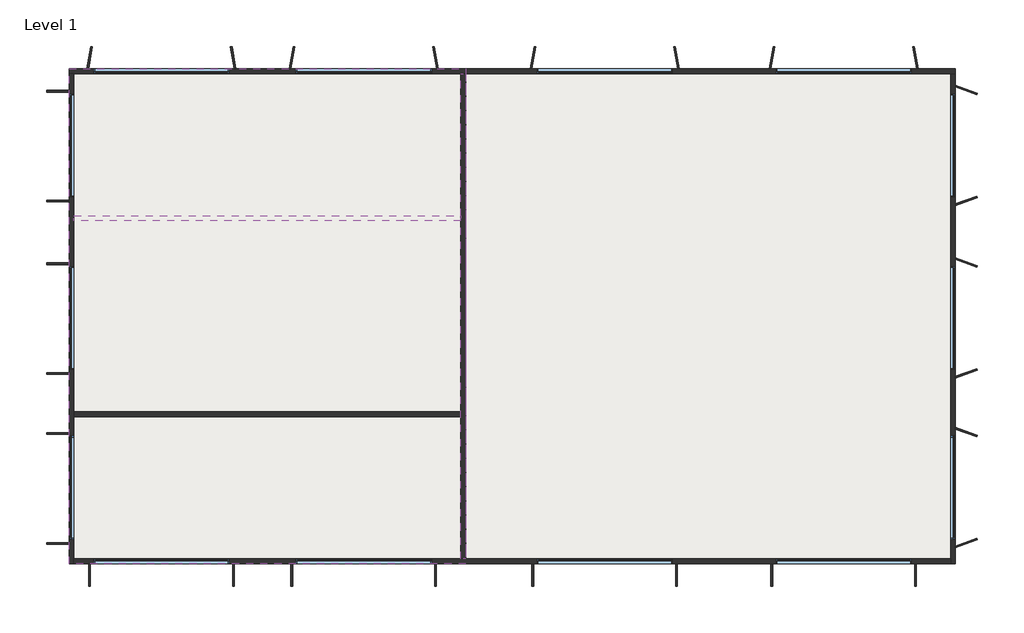
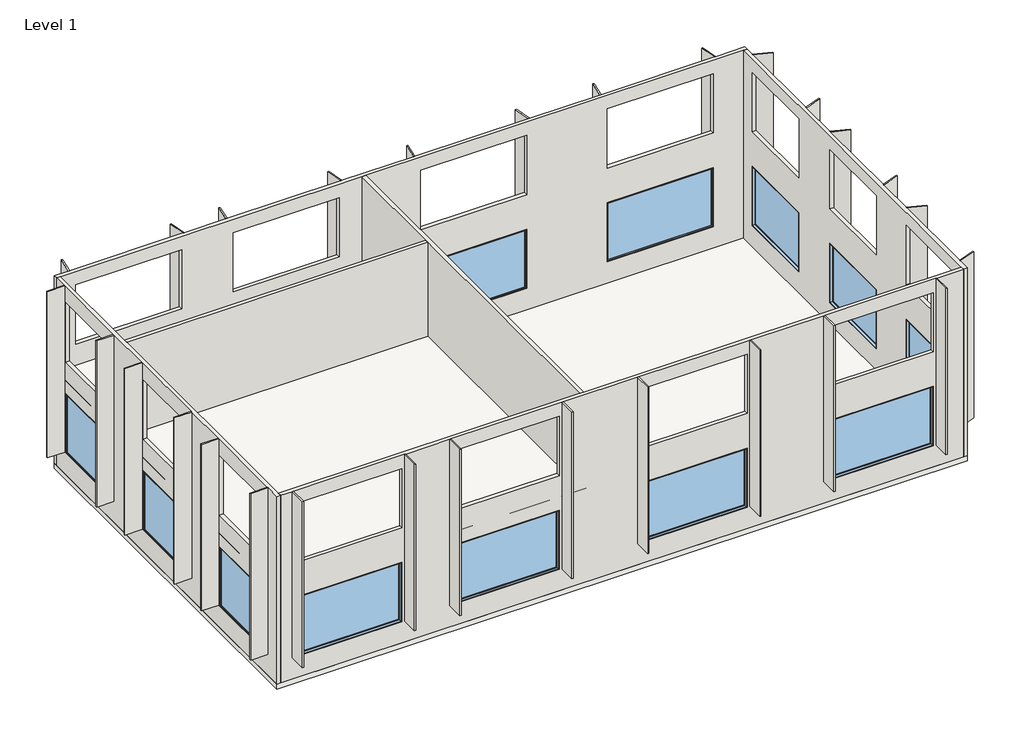
# One storey: 36 walls, 14 windows, 2 slabs.
"""IFC4 building model written with IfcOpenShell, lengths in millimetres."""

import ifcopenshell
import ifcopenshell.guid

model = None  # the IFC model being written
_history = None  # IfcOwnerHistory: only IFC2X3 demands one
_inside = {}  # id of a spatial element -> (the spatial element, [elements in it])
_under = {}  # id of a project, library or spatial element -> (it, [spatial elements below it])
_declared = {}  # id of a project -> (the project, [libraries it declares])
_typed = {}  # id of a type object -> (the type object, [elements of that type])
_made_of = {}  # id of a material, layer set ... -> (it, [elements and type objects made of it])


def new_model(schema):
    """Start an empty IFC model of exactly this schema.

    Asked for "IFC4X3", IfcOpenShell would pick the latest addendum, in which some entities
    have other attributes; the version numbers below select the first issue.
    IFC2X3 requires an IfcOwnerHistory on every rooted entity: one is made here for all.
    """
    global model, _history
    if schema == "IFC4X3":
        model = ifcopenshell.file(schema_version=(4, 3, 0, 0))
    else:
        model = ifcopenshell.file(schema=schema)
    _inside.clear()
    _under.clear()
    _declared.clear()
    _typed.clear()
    _made_of.clear()
    _history = None
    if model.schema == "IFC2X3":
        org = make("IfcOrganization", Name="unknown")
        user = make(
            "IfcPersonAndOrganization",
            ThePerson=make("IfcPerson", FamilyName="unknown"),
            TheOrganization=org,
        )
        app = make(
            "IfcApplication",
            ApplicationDeveloper=org,
            Version="unknown",
            ApplicationFullName="unknown",
            ApplicationIdentifier="unknown",
        )
        _history = make(
            "IfcOwnerHistory",
            OwningUser=user,
            OwningApplication=app,
            ChangeAction="ADDED",
            CreationDate=0,
        )
    return model


def make(cls, **values):
    """One entity of the class cls with the attributes given. An attribute that is None is left unset."""
    return model.create_entity(
        cls, **{name: value for name, value in values.items() if value is not None}
    )


def rooted(cls, **values):
    """An entity with a GlobalId (a new one), such as an element, a storey or a relation."""
    return make(cls, GlobalId=ifcopenshell.guid.new(), OwnerHistory=_history, **values)


def si_unit(unit_type, name, prefix=None):
    """IfcSIUnit, for example si_unit("LENGTHUNIT", "METRE", prefix="MILLI")."""
    return make("IfcSIUnit", UnitType=unit_type, Prefix=prefix, Name=name)


def assignment(units):
    """IfcUnitAssignment: the units of a project."""
    return None if units is None else make("IfcUnitAssignment", Units=units)


def point(xyz):
    """IfcCartesianPoint."""
    return None if xyz is None else make("IfcCartesianPoint", Coordinates=xyz)


def direction(xyz):
    """IfcDirection."""
    return None if xyz is None else make("IfcDirection", DirectionRatios=xyz)


def frame(location, z_axis=None, x_axis=None):
    """IfcAxis2Placement3D, a coordinate frame: its origin and axes. An axis left out is left unset."""
    return make(
        "IfcAxis2Placement3D",
        Location=point(location),
        Axis=direction(z_axis),
        RefDirection=direction(x_axis),
    )


def origin():
    """The frame at (0, 0, 0) with its axes left unset."""
    return frame((0.0, 0.0, 0.0))


def origin_with_axes():
    """The frame at (0, 0, 0) with the z axis (0, 0, 1) and the x axis (1, 0, 0) written out."""
    return frame((0.0, 0.0, 0.0), z_axis=(0.0, 0.0, 1.0), x_axis=(1.0, 0.0, 0.0))


def place(relative_to, where):
    """IfcLocalPlacement: puts the frame where relative to a parent placement (None: the world)."""
    return make(
        "IfcLocalPlacement", PlacementRelTo=relative_to, RelativePlacement=where
    )


def context(
    kind, dimensions, precision=None, world=None, true_north=None, identifier=None
):
    """IfcGeometricRepresentationContext, for example the 3D "Model" context."""
    return make(
        "IfcGeometricRepresentationContext",
        ContextIdentifier=identifier,
        ContextType=kind,
        CoordinateSpaceDimension=dimensions,
        Precision=precision,
        WorldCoordinateSystem=world,
        TrueNorth=true_north,
    )


def project(units=None, contexts=None):
    """IfcProject with its units and contexts."""
    return rooted(
        "IfcProject",
        Name="project",
        RepresentationContexts=contexts,
        UnitsInContext=assignment(units),
    )


def spatial(cls, under=None, at=None, **own):
    """A site, building, storey or space (cls), placed at a placement, below another one or the project."""
    s = rooted(cls, ObjectPlacement=at, **own)
    if under is not None:
        _under.setdefault(under.id(), (under, []))[1].append(s)
    return s


def polyline(points):
    """IfcPolyline through the points."""
    return make("IfcPolyline", Points=[point(p) for p in points])


def outline(outer, holes=None, kind="AREA"):
    """IfcArbitraryClosedProfileDef: a profile drawn as a closed curve; with holes, ...WithVoids."""
    if holes is None:
        return make("IfcArbitraryClosedProfileDef", ProfileType=kind, OuterCurve=outer)
    return make(
        "IfcArbitraryProfileDefWithVoids",
        ProfileType=kind,
        OuterCurve=outer,
        InnerCurves=holes,
    )


def extrude(swept, where, along, depth):
    """IfcExtrudedAreaSolid: the profile swept, set in the frame where, extruded along a direction by depth."""
    return make(
        "IfcExtrudedAreaSolid",
        SweptArea=swept,
        Position=where,
        ExtrudedDirection=direction(along),
        Depth=depth,
    )


def faces_of(points, faces, orient=None, outer=None):
    """IfcFace entities. A face is a list of loops; a loop is a list of indices into points, from 0.

    orient and outer hold one flag for each loop. By default every Orientation is true, the
    first loop of a face is its IfcFaceOuterBound and the others are IfcFaceBound.
    """
    made = []
    for i, loops in enumerate(faces):
        bounds = []
        for j, loop in enumerate(loops):
            is_outer = j == 0 if outer is None else outer[i][j]
            bounds.append(
                make(
                    "IfcFaceOuterBound" if is_outer else "IfcFaceBound",
                    Bound=make("IfcPolyLoop", Polygon=[points[k] for k in loop]),
                    Orientation=True if orient is None else orient[i][j],
                )
            )
        made.append(make("IfcFace", Bounds=bounds))
    return made


def faceted_brep(points, faces, orient=None, outer=None, voids=None):
    """IfcFacetedBrep: a solid bounded by flat faces; with voids (closed shells), ...WithVoids."""
    shared = [point(p) for p in points]
    hull = make("IfcClosedShell", CfsFaces=faces_of(shared, faces, orient, outer))
    if voids is None:
        return make("IfcFacetedBrep", Outer=hull)
    return make(
        "IfcFacetedBrepWithVoids",
        Outer=hull,
        Voids=[
            make(cls, CfsFaces=faces_of(shared, fs, o, b)) for cls, fs, o, b in voids
        ],
    )


def shape(context_of_items, identifier, shape_type, items):
    """IfcShapeRepresentation: the items that make up one representation, for example the "Body"."""
    return make(
        "IfcShapeRepresentation",
        ContextOfItems=context_of_items,
        RepresentationIdentifier=identifier,
        RepresentationType=shape_type,
        Items=items,
    )


def source(mapping_origin, context_of_items, identifier, shape_type, items):
    """IfcRepresentationMap: a shape defined once, which mapped items show again and again."""
    return make(
        "IfcRepresentationMap",
        MappingOrigin=mapping_origin,
        MappedRepresentation=shape(context_of_items, identifier, shape_type, items),
    )


def transform(
    local_origin,
    x_axis=None,
    y_axis=None,
    z_axis=None,
    scale=None,
    scale2=None,
    scale3=None,
    uniform=True,
):
    """IfcCartesianTransformationOperator3D, or its non-uniform kind. x_axis, y_axis, z_axis: its Axis1, 2, 3."""
    if uniform:
        return make(
            "IfcCartesianTransformationOperator3D",
            Axis1=direction(x_axis),
            Axis2=direction(y_axis),
            LocalOrigin=point(local_origin),
            Scale=scale,
            Axis3=direction(z_axis),
        )
    return make(
        "IfcCartesianTransformationOperator3DnonUniform",
        Axis1=direction(x_axis),
        Axis2=direction(y_axis),
        LocalOrigin=point(local_origin),
        Scale=scale,
        Axis3=direction(z_axis),
        Scale2=scale2,
        Scale3=scale3,
    )


def mapped(mapping_source, mapping_target):
    """IfcMappedItem: shows the shape of a source again, moved by a transform."""
    return make(
        "IfcMappedItem", MappingSource=mapping_source, MappingTarget=mapping_target
    )


def made_of(thing, what):
    """Note that an element or type object is made of a material, layer set ...; save() writes the relation."""
    if what is not None:
        _made_of.setdefault(what.id(), (what, []))[1].append(thing)
    return thing


def element(
    cls,
    number,
    at=None,
    inside=None,
    cuts=None,
    type_object=None,
    material=None,
    context=None,
    identifier="Body",
    shape_type=None,
    held_by="IfcProductDefinitionShape",
    body=None,
    shapes=None,
    **own,
):
    """One element of the class cls, such as IfcWall. Its Tag is "e" and its number.

    at: its placement. inside: the storey or other place that contains it. cuts: it is an
    opening in that element (IfcRelVoidsElement). A single representation is given by context,
    identifier, shape_type and body (its items); several are given by shapes. held_by: the class
    of the entity that holds the representations. save() writes the other relations.
    """
    e = rooted(cls, Tag="e%d" % number, ObjectPlacement=at, **own)
    if body is not None:
        shapes = [shape(context, identifier, shape_type, body)]
    if shapes is not None:
        e.Representation = make(held_by, Representations=shapes)
    if inside is not None:
        _inside.setdefault(inside.id(), (inside, []))[1].append(e)
    if cuts is not None:
        rooted(
            "IfcRelVoidsElement", RelatingBuildingElement=cuts, RelatedOpeningElement=e
        )
    if type_object is not None:
        _typed.setdefault(type_object.id(), (type_object, []))[1].append(e)
    return made_of(e, material)


def aggregate(whole, parts):
    """IfcRelAggregates: a whole, such as a stair, and the parts it consists of."""
    return rooted("IfcRelAggregates", RelatingObject=whole, RelatedObjects=parts)


def save(model, path):
    """Write the relations noted so far, then the file.

    IfcRelAggregates (storeys below a building ...), IfcRelContainedInSpatialStructure (elements
    in a storey), IfcRelDefinesByType, IfcRelAssociatesMaterial and IfcRelDeclares: one each for
    every whole, place, type object, material and project.
    """
    for whole, parts in _under.values():
        aggregate(whole, parts)
    for where, things in _inside.values():
        rooted(
            "IfcRelContainedInSpatialStructure",
            RelatedElements=things,
            RelatingStructure=where,
        )
    for kind, things in _typed.values():
        rooted("IfcRelDefinesByType", RelatedObjects=things, RelatingType=kind)
    for what, things in _made_of.values():
        rooted("IfcRelAssociatesMaterial", RelatedObjects=things, RelatingMaterial=what)
    for by, libraries in _declared.values():
        rooted("IfcRelDeclares", RelatingContext=by, RelatedDefinitions=libraries)
    model.write(path)


def m_fixed_2500x_4228mm_fd5e51e7(model_context):
    return source(origin(), model_context, "Body", "SweptSolid", [
        extrude(outline(polyline([(-2050.8, 54.2), (2050.8, 54.2), (2050.8, 42.2), (-2050.8, 42.2), (-2050.8, 54.2)])), frame((0.0, 0.0, 368.0), z_axis=(0.0, 0.0, 1.0), x_axis=(1.0, 0.0, 0.0)), (0.0, 0.0, 1.0), 2374.0),
        extrude(outline(polyline([(2786.0, -2094.8), (324.0, -2094.8), (324.0, 2094.8), (2786.0, 2094.8), (2786.0, -2094.8)]), holes=[polyline([(2742.0, -2050.8), (2742.0, 2050.8), (368.0, 2050.8), (368.0, -2050.8), (2742.0, -2050.8)])]), frame((0.0, 26.2, 0.0), z_axis=(0.0, 1.0, 0.0), x_axis=(0.0, 0.0, 1.0)), (0.0, 0.0, 1.0), 44.0),
        extrude(outline(polyline([(2805.0, -2113.8), (305.0, -2113.8), (305.0, 2113.8), (2805.0, 2113.8), (2805.0, -2113.8)]), holes=[polyline([(2786.0, -2094.8), (2786.0, 2094.8), (324.0, 2094.8), (324.0, -2094.8), (2786.0, -2094.8)])]), frame((0.0, 26.2, 0.0), z_axis=(0.0, 1.0, 0.0), x_axis=(0.0, 0.0, 1.0)), (0.0, 0.0, 1.0), 63.0),
        extrude(outline(polyline([(2805.0, -2113.8), (305.0, -2113.8), (305.0, 2113.8), (2805.0, 2113.8), (2805.0, -2113.8)]), holes=[polyline([(2773.0, -2081.8), (2773.0, 2081.8), (337.0, 2081.8), (337.0, -2081.8), (2773.0, -2081.8)])]), frame((0.0, -63.2, 0.0), z_axis=(0.0, 1.0, 0.0), x_axis=(0.0, 0.0, 1.0)), (0.0, 0.0, 1.0), 89.4),
    ])


def m_fixed_2500x_4228mm_f14c179f(model_context):
    return source(origin(), model_context, "Body", "SweptSolid", [
        extrude(outline(polyline([(-2050.8, -54.2), (-2050.8, -42.2), (2050.8, -42.2), (2050.8, -54.2), (-2050.8, -54.2)])), frame((0.0, 0.0, 368.0), z_axis=(0.0, 0.0, 1.0), x_axis=(1.0, 0.0, 0.0)), (0.0, 0.0, 1.0), 2374.0),
        extrude(outline(polyline([(2786.0, -2094.8), (324.0, -2094.8), (324.0, 2094.8), (2786.0, 2094.8), (2786.0, -2094.8)]), holes=[polyline([(2742.0, -2050.8), (2742.0, 2050.8), (368.0, 2050.8), (368.0, -2050.8), (2742.0, -2050.8)])]), frame((0.0, -70.2, 0.0), z_axis=(0.0, 1.0, 0.0), x_axis=(0.0, 0.0, 1.0)), (0.0, 0.0, 1.0), 44.0),
        extrude(outline(polyline([(2805.0, -2113.8), (305.0, -2113.8), (305.0, 2113.8), (2805.0, 2113.8), (2805.0, -2113.8)]), holes=[polyline([(2786.0, -2094.8), (2786.0, 2094.8), (324.0, 2094.8), (324.0, -2094.8), (2786.0, -2094.8)])]), frame((0.0, -89.2, 0.0), z_axis=(0.0, 1.0, 0.0), x_axis=(0.0, 0.0, 1.0)), (0.0, 0.0, 1.0), 63.0),
        extrude(outline(polyline([(2805.0, -2113.8), (305.0, -2113.8), (305.0, 2113.8), (2805.0, 2113.8), (2805.0, -2113.8)]), holes=[polyline([(2773.0, -2081.8), (2773.0, 2081.8), (337.0, 2081.8), (337.0, -2081.8), (2773.0, -2081.8)])]), frame((0.0, -26.2, 0.0), z_axis=(0.0, 1.0, 0.0), x_axis=(0.0, 0.0, 1.0)), (0.0, 0.0, 1.0), 89.4),
    ])


def m_fixed_2500x_3220mm_df94f4d0(model_context):
    return source(origin(), model_context, "Body", "SweptSolid", [
        extrude(outline(polyline([(-1546.8, 54.2), (1546.8, 54.2), (1546.8, 42.2), (-1546.8, 42.2), (-1546.8, 54.2)])), frame((0.0, 0.0, 368.0), z_axis=(0.0, 0.0, 1.0), x_axis=(1.0, 0.0, 0.0)), (0.0, 0.0, 1.0), 2374.0),
        extrude(outline(polyline([(2786.0, -1590.8), (324.0, -1590.8), (324.0, 1590.8), (2786.0, 1590.8), (2786.0, -1590.8)]), holes=[polyline([(2742.0, -1546.8), (2742.0, 1546.8), (368.0, 1546.8), (368.0, -1546.8), (2742.0, -1546.8)])]), frame((0.0, 26.2, 0.0), z_axis=(0.0, 1.0, 0.0), x_axis=(0.0, 0.0, 1.0)), (0.0, 0.0, 1.0), 44.0),
        extrude(outline(polyline([(2805.0, -1609.8), (305.0, -1609.8), (305.0, 1609.8), (2805.0, 1609.8), (2805.0, -1609.8)]), holes=[polyline([(2786.0, -1590.8), (2786.0, 1590.8), (324.0, 1590.8), (324.0, -1590.8), (2786.0, -1590.8)])]), frame((0.0, 26.2, 0.0), z_axis=(0.0, 1.0, 0.0), x_axis=(0.0, 0.0, 1.0)), (0.0, 0.0, 1.0), 63.0),
        extrude(outline(polyline([(2805.0, -1609.8), (305.0, -1609.8), (305.0, 1609.8), (2805.0, 1609.8), (2805.0, -1609.8)]), holes=[polyline([(2773.0, -1577.8), (2773.0, 1577.8), (337.0, 1577.8), (337.0, -1577.8), (2773.0, -1577.8)])]), frame((0.0, -63.2, 0.0), z_axis=(0.0, 1.0, 0.0), x_axis=(0.0, 0.0, 1.0)), (0.0, 0.0, 1.0), 89.4),
    ])


def m_fixed_2500x_3220mm_8b997f8c(model_context):
    return source(origin(), model_context, "Body", "SweptSolid", [
        extrude(outline(polyline([(-1546.8, -54.2), (-1546.8, -42.2), (1546.8, -42.2), (1546.8, -54.2), (-1546.8, -54.2)])), frame((0.0, 0.0, 368.0), z_axis=(0.0, 0.0, 1.0), x_axis=(1.0, 0.0, 0.0)), (0.0, 0.0, 1.0), 2374.0),
        extrude(outline(polyline([(2786.0, -1590.8), (324.0, -1590.8), (324.0, 1590.8), (2786.0, 1590.8), (2786.0, -1590.8)]), holes=[polyline([(2742.0, -1546.8), (2742.0, 1546.8), (368.0, 1546.8), (368.0, -1546.8), (2742.0, -1546.8)])]), frame((0.0, -70.2, 0.0), z_axis=(0.0, 1.0, 0.0), x_axis=(0.0, 0.0, 1.0)), (0.0, 0.0, 1.0), 44.0),
        extrude(outline(polyline([(2805.0, -1609.8), (305.0, -1609.8), (305.0, 1609.8), (2805.0, 1609.8), (2805.0, -1609.8)]), holes=[polyline([(2786.0, -1590.8), (2786.0, 1590.8), (324.0, 1590.8), (324.0, -1590.8), (2786.0, -1590.8)])]), frame((0.0, -89.2, 0.0), z_axis=(0.0, 1.0, 0.0), x_axis=(0.0, 0.0, 1.0)), (0.0, 0.0, 1.0), 63.0),
        extrude(outline(polyline([(2805.0, -1609.8), (305.0, -1609.8), (305.0, 1609.8), (2805.0, 1609.8), (2805.0, -1609.8)]), holes=[polyline([(2773.0, -1577.8), (2773.0, 1577.8), (337.0, 1577.8), (337.0, -1577.8), (2773.0, -1577.8)])]), frame((0.0, -26.2, 0.0), z_axis=(0.0, 1.0, 0.0), x_axis=(0.0, 0.0, 1.0)), (0.0, 0.0, 1.0), 89.4),
    ])


model = new_model("IFC4")

# Units and contexts
model_context = context("Model", 3, world=origin())
ifc_project = project(units=[si_unit("LENGTHUNIT", "METRE", prefix="MILLI")], contexts=[model_context])

# Site, building, storey
site = spatial("IfcSite", under=ifc_project)
building = spatial("IfcBuilding", under=site)
storey = spatial("IfcBuildingStorey", under=building, Name="Level 1", Elevation=0.0)

# Slabs
placement = place(None, origin())
element("IfcSlab", 1, ObjectType="160mm Concrete With 50mm Metal Deck", at=placement, inside=storey, context=model_context, shape_type="Brep", body=[
    faceted_brep([(29068.464681, 11296.9802217, -210.0), (29068.464681, -4095.4197783, -210.0), (1484.064681, -4095.4197783, -210.0), (1484.064681, 11296.9802217, -210.0), (29068.464681, 11296.9802217, 0.0), (1484.064681, 11296.9802217, 0.0), (1484.064681, -4095.4197783, 0.0), (28916.064681, -4095.4197783, 0.0), (29068.464681, -4095.4197783, 0.0), (29068.464681, 11144.5802217, 0.0)], [[[0, 1, 2, 3]], [[4, 5, 6, 7, 8, 9]], [[1, 0, 4, 9, 8]], [[2, 1, 8, 7, 6]], [[3, 2, 6, 5]], [[0, 3, 5, 4]]]),
])
element("IfcSlab", 2, ObjectType="160mm Concrete With 50mm Metal Deck", at=placement, inside=storey, context=model_context, shape_type="SweptSolid", body=[
    extrude(outline(polyline([(13828.464681, 11296.9802217), (13828.464681, -4095.4197783), (1484.064681, -4095.4197783), (1484.064681, 11296.9802217), (13828.464681, 11296.9802217)])), frame((0.0, 0.0, 3752.4), z_axis=(0.0, 0.0, 1.0), x_axis=(1.0, 0.0, 0.0)), (0.0, 0.0, 1.0), 210.0),
])

# Walls
element("IfcWall", 3, ObjectType="Generic - 152.4mm", at=placement, inside=storey, context=model_context, shape_type="Brep", body=[
    faceted_brep([(1484.064681, 11144.5802217, 0.0), (1636.464681, 11144.5802217, 0.0), (13676.064681, 11144.5802217, 0.0), (13828.464681, 11144.5802217, 0.0), (28916.064681, 11144.5802217, 0.0), (29068.464681, 11144.5802217, 0.0), (29068.464681, 11144.5802217, 7924.8), (28916.064681, 11144.5802217, 7924.8), (13828.464681, 11144.5802217, 7924.8), (13676.064681, 11144.5802217, 7924.8), (1636.464681, 11144.5802217, 7924.8), (1484.064681, 11144.5802217, 7924.8), (6474.064681, 11144.5802217, 902.4), (2246.464681, 11144.5802217, 902.4), (2246.464681, 11144.5802217, 3402.4), (6474.064681, 11144.5802217, 3402.4), (12766.064681, 11144.5802217, 902.4), (8538.464681, 11144.5802217, 902.4), (8538.464681, 11144.5802217, 3402.4), (12766.064681, 11144.5802217, 3402.4), (20266.064681, 11144.5802217, 902.4), (16038.464681, 11144.5802217, 902.4), (16038.464681, 11144.5802217, 3402.4), (20266.064681, 11144.5802217, 3402.4), (27706.064681, 11144.5802217, 902.4), (23478.464681, 11144.5802217, 902.4), (23478.464681, 11144.5802217, 3402.4), (27706.064681, 11144.5802217, 3402.4), (27706.064681, 11144.5802217, 4862.4), (23478.464681, 11144.5802217, 4862.4), (23478.464681, 11144.5802217, 7362.4), (27706.064681, 11144.5802217, 7362.4), (20266.064681, 11144.5802217, 4862.4), (16038.464681, 11144.5802217, 4862.4), (16038.464681, 11144.5802217, 7362.4), (20266.064681, 11144.5802217, 7362.4), (12766.064681, 11144.5802217, 4862.4), (8538.464681, 11144.5802217, 4862.4), (8538.464681, 11144.5802217, 7362.4), (12766.064681, 11144.5802217, 7362.4), (6474.064681, 11144.5802217, 4862.4), (2246.464681, 11144.5802217, 4862.4), (2246.464681, 11144.5802217, 7362.4), (6474.064681, 11144.5802217, 7362.4), (1484.064681, 11296.9802217, 0.0), (1484.064681, 11296.9802217, 7924.8), (2041.0826304, 11296.9802217, 7924.8), (2091.853961, 11296.9802217, 7924.8), (6628.675401, 11296.9802217, 7924.8), (6679.4467316, 11296.9802217, 7924.8), (8333.0826304, 11296.9802217, 7924.8), (8383.853961, 11296.9802217, 7924.8), (12920.675401, 11296.9802217, 7924.8), (12971.4467316, 11296.9802217, 7924.8), (15833.0826304, 11296.9802217, 7924.8), (15883.853961, 11296.9802217, 7924.8), (20420.675401, 11296.9802217, 7924.8), (20471.4467316, 11296.9802217, 7924.8), (23273.0826304, 11296.9802217, 7924.8), (23323.853961, 11296.9802217, 7924.8), (27860.675401, 11296.9802217, 7924.8), (27911.4467316, 11296.9802217, 7924.8), (29068.464681, 11296.9802217, 7924.8), (29068.464681, 11296.9802217, 0.0), (6474.064681, 11296.9802217, 902.4), (6474.064681, 11296.9802217, 3402.4), (2246.464681, 11296.9802217, 3402.4), (2246.464681, 11296.9802217, 902.4), (12766.064681, 11296.9802217, 902.4), (12766.064681, 11296.9802217, 3402.4), (8538.464681, 11296.9802217, 3402.4), (8538.464681, 11296.9802217, 902.4), (20266.064681, 11296.9802217, 902.4), (20266.064681, 11296.9802217, 3402.4), (16038.464681, 11296.9802217, 3402.4), (16038.464681, 11296.9802217, 902.4), (27706.064681, 11296.9802217, 902.4), (27706.064681, 11296.9802217, 3402.4), (23478.464681, 11296.9802217, 3402.4), (23478.464681, 11296.9802217, 902.4), (27706.064681, 11296.9802217, 4862.4), (27706.064681, 11296.9802217, 7362.4), (23478.464681, 11296.9802217, 7362.4), (23478.464681, 11296.9802217, 4862.4), (20266.064681, 11296.9802217, 4862.4), (20266.064681, 11296.9802217, 7362.4), (16038.464681, 11296.9802217, 7362.4), (16038.464681, 11296.9802217, 4862.4), (12766.064681, 11296.9802217, 4862.4), (12766.064681, 11296.9802217, 7362.4), (8538.464681, 11296.9802217, 7362.4), (8538.464681, 11296.9802217, 4862.4), (6474.064681, 11296.9802217, 4862.4), (6474.064681, 11296.9802217, 7362.4), (2246.464681, 11296.9802217, 7362.4), (2246.464681, 11296.9802217, 4862.4)], [[[0, 1, 2, 3, 4, 5, 6, 7, 8, 9, 10, 11], [12, 13, 14, 15], [16, 17, 18, 19], [20, 21, 22, 23], [24, 25, 26, 27], [28, 29, 30, 31], [32, 33, 34, 35], [36, 37, 38, 39], [40, 41, 42, 43]], [[44, 45, 46, 47, 48, 49, 50, 51, 52, 53, 54, 55, 56, 57, 58, 59, 60, 61, 62, 63], [64, 65, 66, 67], [68, 69, 70, 71], [72, 73, 74, 75], [76, 77, 78, 79], [80, 81, 82, 83], [84, 85, 86, 87], [88, 89, 90, 91], [92, 93, 94, 95]], [[5, 4, 3, 2, 1, 0, 44, 63]], [[11, 10, 9, 8, 7, 6, 62, 61, 60, 59, 58, 57, 56, 55, 54, 53, 52, 51, 50, 49, 48, 47, 46, 45]], [[6, 5, 63, 62]], [[0, 11, 45, 44]], [[65, 64, 12, 15]], [[66, 65, 15, 14]], [[67, 66, 14, 13]], [[64, 67, 13, 12]], [[69, 68, 16, 19]], [[70, 69, 19, 18]], [[71, 70, 18, 17]], [[68, 71, 17, 16]], [[73, 72, 20, 23]], [[74, 73, 23, 22]], [[75, 74, 22, 21]], [[72, 75, 21, 20]], [[77, 76, 24, 27]], [[78, 77, 27, 26]], [[79, 78, 26, 25]], [[76, 79, 25, 24]], [[81, 80, 28, 31]], [[82, 81, 31, 30]], [[83, 82, 30, 29]], [[80, 83, 29, 28]], [[85, 84, 32, 35]], [[86, 85, 35, 34]], [[87, 86, 34, 33]], [[84, 87, 33, 32]], [[89, 88, 36, 39]], [[90, 89, 39, 38]], [[91, 90, 38, 37]], [[88, 91, 37, 36]], [[93, 92, 40, 43]], [[94, 93, 43, 42]], [[95, 94, 42, 41]], [[92, 95, 41, 40]]]),
])
element("IfcWall", 4, ObjectType="Generic - 152.4mm", at=placement, inside=storey, context=model_context, shape_type="Brep", body=[
    faceted_brep([(28916.064681, 11144.5802217, 0.0), (28916.064681, -3943.0197783, 0.0), (28916.064681, -4095.4197783, 0.0), (28916.064681, -4095.4197783, 7924.8), (28916.064681, -3943.0197783, 7924.8), (28916.064681, 11144.5802217, 7924.8), (28916.064681, -3343.0197783, 902.4), (28916.064681, -123.4197783, 902.4), (28916.064681, -123.4197783, 3402.4), (28916.064681, -3343.0197783, 3402.4), (28916.064681, 1942.9802217, 902.4), (28916.064681, 5162.5802217, 902.4), (28916.064681, 5162.5802217, 3402.4), (28916.064681, 1942.9802217, 3402.4), (28916.064681, 7310.9802217, 902.4), (28916.064681, 10530.5802217, 902.4), (28916.064681, 10530.5802217, 3402.4), (28916.064681, 7310.9802217, 3402.4), (28916.064681, -3343.0197783, 4864.8), (28916.064681, -123.4197783, 4864.8), (28916.064681, -123.4197783, 7364.8), (28916.064681, -3343.0197783, 7364.8), (28916.064681, 1942.9802217, 4864.8), (28916.064681, 5162.5802217, 4864.8), (28916.064681, 5162.5802217, 7364.8), (28916.064681, 1942.9802217, 7364.8), (28916.064681, 7310.9802217, 4864.8), (28916.064681, 10530.5802217, 4864.8), (28916.064681, 10530.5802217, 7364.8), (28916.064681, 7310.9802217, 7364.8), (29068.464681, 11144.5802217, 0.0), (29068.464681, 11144.5802217, 7924.8), (29068.464681, 10795.706982, 7924.8), (29068.464681, 10742.4980934, 7924.8), (29068.464681, 7099.0623499, 7924.8), (29068.464681, 7045.8534613, 7924.8), (29068.464681, 5427.706982, 7924.8), (29068.464681, 5374.4980934, 7924.8), (29068.464681, 1731.0623499, 7924.8), (29068.464681, 1677.8534613, 7924.8), (29068.464681, 141.706982, 7924.8), (29068.464681, 88.4980934, 7924.8), (29068.464681, -3554.9376501, 7924.8), (29068.464681, -3608.1465387, 7924.8), (29068.464681, -4095.4197783, 7924.8), (29068.464681, -4095.4197783, 0.0), (29068.464681, -3343.0197783, 902.4), (29068.464681, -3343.0197783, 3402.4), (29068.464681, -123.4197783, 3402.4), (29068.464681, -123.4197783, 902.4), (29068.464681, 1942.9802217, 902.4), (29068.464681, 1942.9802217, 3402.4), (29068.464681, 5162.5802217, 3402.4), (29068.464681, 5162.5802217, 902.4), (29068.464681, 7310.9802217, 902.4), (29068.464681, 7310.9802217, 3402.4), (29068.464681, 10530.5802217, 3402.4), (29068.464681, 10530.5802217, 902.4), (29068.464681, -3343.0197783, 4864.8), (29068.464681, -3343.0197783, 7364.8), (29068.464681, -123.4197783, 7364.8), (29068.464681, -123.4197783, 4864.8), (29068.464681, 1942.9802217, 4864.8), (29068.464681, 1942.9802217, 7364.8), (29068.464681, 5162.5802217, 7364.8), (29068.464681, 5162.5802217, 4864.8), (29068.464681, 7310.9802217, 4864.8), (29068.464681, 7310.9802217, 7364.8), (29068.464681, 10530.5802217, 7364.8), (29068.464681, 10530.5802217, 4864.8)], [[[0, 1, 2, 3, 4, 5], [6, 7, 8, 9], [10, 11, 12, 13], [14, 15, 16, 17], [18, 19, 20, 21], [22, 23, 24, 25], [26, 27, 28, 29]], [[30, 31, 32, 33, 34, 35, 36, 37, 38, 39, 40, 41, 42, 43, 44, 45], [46, 47, 48, 49], [50, 51, 52, 53], [54, 55, 56, 57], [58, 59, 60, 61], [62, 63, 64, 65], [66, 67, 68, 69]], [[2, 1, 0, 30, 45]], [[5, 4, 3, 44, 43, 42, 41, 40, 39, 38, 37, 36, 35, 34, 33, 32, 31]], [[0, 5, 31, 30]], [[47, 46, 6, 9]], [[48, 47, 9, 8]], [[49, 48, 8, 7]], [[46, 49, 7, 6]], [[51, 50, 10, 13]], [[52, 51, 13, 12]], [[53, 52, 12, 11]], [[50, 53, 11, 10]], [[55, 54, 14, 17]], [[56, 55, 17, 16]], [[57, 56, 16, 15]], [[54, 57, 15, 14]], [[3, 2, 45, 44]], [[59, 58, 18, 21]], [[60, 59, 21, 20]], [[61, 60, 20, 19]], [[58, 61, 19, 18]], [[63, 62, 22, 25]], [[64, 63, 25, 24]], [[65, 64, 24, 23]], [[62, 65, 23, 22]], [[67, 66, 26, 29]], [[68, 67, 29, 28]], [[69, 68, 28, 27]], [[66, 69, 27, 26]]]),
])
element("IfcWall", 5, ObjectType="Generic - 152.4mm", at=placement, inside=storey, context=model_context, shape_type="Brep", body=[
    faceted_brep([(28916.064681, -3943.0197783, 0.0), (13828.464681, -3943.0197783, 0.0), (13676.064681, -3943.0197783, 0.0), (1636.464681, -3943.0197783, 0.0), (1636.464681, -3943.0197783, 7924.8), (13676.064681, -3943.0197783, 7924.8), (13828.464681, -3943.0197783, 7924.8), (28916.064681, -3943.0197783, 7924.8), (27706.064681, -3943.0197783, 902.4), (27706.064681, -3943.0197783, 3402.4), (23478.464681, -3943.0197783, 3402.4), (23478.464681, -3943.0197783, 902.4), (20266.064681, -3943.0197783, 902.4), (20266.064681, -3943.0197783, 3402.4), (16038.464681, -3943.0197783, 3402.4), (16038.464681, -3943.0197783, 902.4), (12766.064681, -3943.0197783, 902.4), (12766.064681, -3943.0197783, 3402.4), (8538.464681, -3943.0197783, 3402.4), (8538.464681, -3943.0197783, 902.4), (6474.064681, -3943.0197783, 902.4), (6474.064681, -3943.0197783, 3402.4), (2246.464681, -3943.0197783, 3402.4), (2246.464681, -3943.0197783, 902.4), (27706.064681, -3943.0197783, 4862.4), (27706.064681, -3943.0197783, 7362.4), (23478.464681, -3943.0197783, 7362.4), (23478.464681, -3943.0197783, 4862.4), (20266.064681, -3943.0197783, 4862.4), (20266.064681, -3943.0197783, 7362.4), (16038.464681, -3943.0197783, 7362.4), (16038.464681, -3943.0197783, 4862.4), (12766.064681, -3943.0197783, 4862.4), (12766.064681, -3943.0197783, 7362.4), (8538.464681, -3943.0197783, 7362.4), (8538.464681, -3943.0197783, 4862.4), (6474.064681, -3943.0197783, 4862.4), (6474.064681, -3943.0197783, 7362.4), (2246.464681, -3943.0197783, 7362.4), (2246.464681, -3943.0197783, 4862.4), (28916.064681, -4095.4197783, 0.0), (28916.064681, -4095.4197783, 7924.8), (27856.064681, -4095.4197783, 7924.8), (27806.064681, -4095.4197783, 7924.8), (23378.464681, -4095.4197783, 7924.8), (23328.464681, -4095.4197783, 7924.8), (20416.064681, -4095.4197783, 7924.8), (20366.064681, -4095.4197783, 7924.8), (15938.464681, -4095.4197783, 7924.8), (15888.464681, -4095.4197783, 7924.8), (12916.064681, -4095.4197783, 7924.8), (12866.064681, -4095.4197783, 7924.8), (8438.464681, -4095.4197783, 7924.8), (8388.464681, -4095.4197783, 7924.8), (6624.064681, -4095.4197783, 7924.8), (6574.064681, -4095.4197783, 7924.8), (2146.464681, -4095.4197783, 7924.8), (2096.464681, -4095.4197783, 7924.8), (1636.464681, -4095.4197783, 7924.8), (1636.464681, -4095.4197783, 0.0), (27706.064681, -4095.4197783, 902.4), (23478.464681, -4095.4197783, 902.4), (23478.464681, -4095.4197783, 3402.4), (27706.064681, -4095.4197783, 3402.4), (20266.064681, -4095.4197783, 902.4), (16038.464681, -4095.4197783, 902.4), (16038.464681, -4095.4197783, 3402.4), (20266.064681, -4095.4197783, 3402.4), (12766.064681, -4095.4197783, 902.4), (8538.464681, -4095.4197783, 902.4), (8538.464681, -4095.4197783, 3402.4), (12766.064681, -4095.4197783, 3402.4), (6474.064681, -4095.4197783, 902.4), (2246.464681, -4095.4197783, 902.4), (2246.464681, -4095.4197783, 3402.4), (6474.064681, -4095.4197783, 3402.4), (27706.064681, -4095.4197783, 4862.4), (23478.464681, -4095.4197783, 4862.4), (23478.464681, -4095.4197783, 7362.4), (27706.064681, -4095.4197783, 7362.4), (20266.064681, -4095.4197783, 4862.4), (16038.464681, -4095.4197783, 4862.4), (16038.464681, -4095.4197783, 7362.4), (20266.064681, -4095.4197783, 7362.4), (12766.064681, -4095.4197783, 4862.4), (8538.464681, -4095.4197783, 4862.4), (8538.464681, -4095.4197783, 7362.4), (12766.064681, -4095.4197783, 7362.4), (6474.064681, -4095.4197783, 4862.4), (2246.464681, -4095.4197783, 4862.4), (2246.464681, -4095.4197783, 7362.4), (6474.064681, -4095.4197783, 7362.4)], [[[0, 1, 2, 3, 4, 5, 6, 7], [8, 9, 10, 11], [12, 13, 14, 15], [16, 17, 18, 19], [20, 21, 22, 23], [24, 25, 26, 27], [28, 29, 30, 31], [32, 33, 34, 35], [36, 37, 38, 39]], [[40, 41, 42, 43, 44, 45, 46, 47, 48, 49, 50, 51, 52, 53, 54, 55, 56, 57, 58, 59], [60, 61, 62, 63], [64, 65, 66, 67], [68, 69, 70, 71], [72, 73, 74, 75], [76, 77, 78, 79], [80, 81, 82, 83], [84, 85, 86, 87], [88, 89, 90, 91]], [[3, 2, 1, 0, 40, 59]], [[7, 6, 5, 4, 58, 57, 56, 55, 54, 53, 52, 51, 50, 49, 48, 47, 46, 45, 44, 43, 42, 41]], [[9, 8, 60, 63]], [[10, 9, 63, 62]], [[11, 10, 62, 61]], [[8, 11, 61, 60]], [[13, 12, 64, 67]], [[14, 13, 67, 66]], [[15, 14, 66, 65]], [[12, 15, 65, 64]], [[17, 16, 68, 71]], [[18, 17, 71, 70]], [[19, 18, 70, 69]], [[16, 19, 69, 68]], [[21, 20, 72, 75]], [[22, 21, 75, 74]], [[23, 22, 74, 73]], [[20, 23, 73, 72]], [[0, 7, 41, 40]], [[4, 3, 59, 58]], [[25, 24, 76, 79]], [[26, 25, 79, 78]], [[27, 26, 78, 77]], [[24, 27, 77, 76]], [[29, 28, 80, 83]], [[30, 29, 83, 82]], [[31, 30, 82, 81]], [[28, 31, 81, 80]], [[33, 32, 84, 87]], [[34, 33, 87, 86]], [[35, 34, 86, 85]], [[32, 35, 85, 84]], [[37, 36, 88, 91]], [[38, 37, 91, 90]], [[39, 38, 90, 89]], [[36, 39, 89, 88]]]),
])
element("IfcWall", 6, ObjectType="Generic - 152.4mm", at=placement, inside=storey, context=model_context, shape_type="Brep", body=[
    faceted_brep([(1636.464681, -4095.4197783, 0.0), (1636.464681, -3943.0197783, 0.0), (1636.464681, 476.5802217, 0.0), (1636.464681, 628.9802217, 0.0), (1636.464681, 11144.5802217, 0.0), (1636.464681, 11144.5802217, 7924.8), (1636.464681, 6724.9802217, 7924.8), (1636.464681, 6572.5802217, 7924.8), (1636.464681, -3943.0197783, 7924.8), (1636.464681, -4095.4197783, 7924.8), (1636.464681, 7310.9802217, 4734.5029682), (1636.464681, 7310.9802217, 7234.5029682), (1636.464681, 10530.5802217, 7234.5029682), (1636.464681, 10530.5802217, 4734.5029682), (1636.464681, 1942.9802217, 4734.5029682), (1636.464681, 1942.9802217, 7234.5029682), (1636.464681, 5162.5802217, 7234.5029682), (1636.464681, 5162.5802217, 4734.5029682), (1636.464681, -3343.0197783, 4734.5029682), (1636.464681, -3343.0197783, 7234.5029682), (1636.464681, -123.4197783, 7234.5029682), (1636.464681, -123.4197783, 4734.5029682), (1636.464681, -3343.0197783, 902.4), (1636.464681, -3343.0197783, 3402.4), (1636.464681, -123.4197783, 3402.4), (1636.464681, -123.4197783, 902.4), (1636.464681, 7310.9802217, 902.4), (1636.464681, 7310.9802217, 3402.4), (1636.464681, 10530.5802217, 3402.4), (1636.464681, 10530.5802217, 902.4), (1636.464681, 1942.9802217, 902.4), (1636.464681, 1942.9802217, 3402.4), (1636.464681, 5162.5802217, 3402.4), (1636.464681, 5162.5802217, 902.4), (1484.064681, -4095.4197783, 0.0), (1484.064681, -4095.4197783, 7924.8), (1484.064681, -3493.0197783, 7924.8), (1484.064681, -3443.0197783, 7924.8), (1484.064681, -73.4197783, 7924.8), (1484.064681, -23.4197783, 7924.8), (1484.064681, 1792.9802217, 7924.8), (1484.064681, 1842.9802217, 7924.8), (1484.064681, 5212.5802217, 7924.8), (1484.064681, 5262.5802217, 7924.8), (1484.064681, 7160.9802217, 7924.8), (1484.064681, 7210.9802217, 7924.8), (1484.064681, 10580.5802217, 7924.8), (1484.064681, 10630.5802217, 7924.8), (1484.064681, 11144.5802217, 7924.8), (1484.064681, 11144.5802217, 0.0), (1484.064681, 7310.9802217, 4734.5029682), (1484.064681, 10530.5802217, 4734.5029682), (1484.064681, 10530.5802217, 7234.5029682), (1484.064681, 7310.9802217, 7234.5029682), (1484.064681, 1942.9802217, 4734.5029682), (1484.064681, 5162.5802217, 4734.5029682), (1484.064681, 5162.5802217, 7234.5029682), (1484.064681, 1942.9802217, 7234.5029682), (1484.064681, -3343.0197783, 4734.5029682), (1484.064681, -123.4197783, 4734.5029682), (1484.064681, -123.4197783, 7234.5029682), (1484.064681, -3343.0197783, 7234.5029682), (1484.064681, -3343.0197783, 902.4), (1484.064681, -123.4197783, 902.4), (1484.064681, -123.4197783, 3402.4), (1484.064681, -3343.0197783, 3402.4), (1484.064681, 7310.9802217, 902.4), (1484.064681, 10530.5802217, 902.4), (1484.064681, 10530.5802217, 3402.4), (1484.064681, 7310.9802217, 3402.4), (1484.064681, 1942.9802217, 902.4), (1484.064681, 5162.5802217, 902.4), (1484.064681, 5162.5802217, 3402.4), (1484.064681, 1942.9802217, 3402.4)], [[[0, 1, 2, 3, 4, 5, 6, 7, 8, 9], [10, 11, 12, 13], [14, 15, 16, 17], [18, 19, 20, 21], [22, 23, 24, 25], [26, 27, 28, 29], [30, 31, 32, 33]], [[34, 35, 36, 37, 38, 39, 40, 41, 42, 43, 44, 45, 46, 47, 48, 49], [50, 51, 52, 53], [54, 55, 56, 57], [58, 59, 60, 61], [62, 63, 64, 65], [66, 67, 68, 69], [70, 71, 72, 73]], [[4, 3, 2, 1, 0, 34, 49]], [[9, 8, 7, 6, 5, 48, 47, 46, 45, 44, 43, 42, 41, 40, 39, 38, 37, 36, 35]], [[5, 4, 49, 48]], [[0, 9, 35, 34]], [[11, 10, 50, 53]], [[12, 11, 53, 52]], [[13, 12, 52, 51]], [[10, 13, 51, 50]], [[15, 14, 54, 57]], [[16, 15, 57, 56]], [[17, 16, 56, 55]], [[14, 17, 55, 54]], [[19, 18, 58, 61]], [[20, 19, 61, 60]], [[21, 20, 60, 59]], [[18, 21, 59, 58]], [[23, 22, 62, 65]], [[24, 23, 65, 64]], [[25, 24, 64, 63]], [[22, 25, 63, 62]], [[27, 26, 66, 69]], [[28, 27, 69, 68]], [[29, 28, 68, 67]], [[26, 29, 67, 66]], [[31, 30, 70, 73]], [[32, 31, 73, 72]], [[33, 32, 72, 71]], [[30, 33, 71, 70]]]),
])
element("IfcWall", 7, ObjectType="Generic - 152.4mm - Interior", at=placement, inside=storey, context=model_context, shape_type="Brep", body=[
    faceted_brep([(13828.464681, -3943.0197783, 0.0), (13828.464681, 11144.5802217, 0.0), (13828.464681, 11144.5802217, 3752.4), (13828.464681, -3943.0197783, 3752.4), (13676.064681, -3943.0197783, 0.0), (13676.064681, -3943.0197783, 3752.4), (13676.064681, 476.5802217, 3752.4), (13676.064681, 628.9802217, 3752.4), (13676.064681, 11144.5802217, 3752.4), (13676.064681, 11144.5802217, 0.0), (13676.064681, 628.9802217, 0.0), (13676.064681, 476.5802217, 0.0)], [[[0, 1, 2, 3]], [[4, 5, 6, 7, 8, 9, 10, 11]], [[1, 0, 4, 11, 10, 9]], [[0, 3, 5, 4]], [[2, 1, 9, 8]], [[3, 2, 8, 7, 6, 5]]]),
])
element("IfcWall", 8, ObjectType="Generic - 152.4mm - Interior", at=placement, inside=storey, context=model_context, shape_type="SweptSolid", body=[
    extrude(outline(polyline([(1636.464681, 628.9802217), (13676.064681, 628.9802217), (13676.064681, 476.5802217), (1636.464681, 476.5802217), (1636.464681, 628.9802217)])), origin_with_axes(), (0.0, 0.0, 1.0), 3752.4),
])
element("IfcWall", 9, ObjectType="Generic - 152.4mm - Interior", at=placement, inside=storey, context=model_context, shape_type="Brep", body=[
    faceted_brep([(13676.064681, 11144.5802217, 3962.4), (13676.064681, 6724.9802217, 3962.4), (13676.064681, 6572.5802217, 3962.4), (13676.064681, -3943.0197783, 3962.4), (13676.064681, -3943.0197783, 7924.8), (13676.064681, 6572.5802217, 7924.8), (13676.064681, 6724.9802217, 7924.8), (13676.064681, 11144.5802217, 7924.8), (13828.464681, 11144.5802217, 3962.4), (13828.464681, 11144.5802217, 7924.8), (13828.464681, -3943.0197783, 7924.8), (13828.464681, -3943.0197783, 3962.4)], [[[0, 1, 2, 3, 4, 5, 6, 7]], [[8, 9, 10, 11]], [[3, 2, 1, 0, 8, 11]], [[7, 6, 5, 4, 10, 9]], [[4, 3, 11, 10]], [[0, 7, 9, 8]]]),
])
element("IfcWall", 10, ObjectType="Generic - 152.4mm - Interior", at=placement, inside=storey, context=model_context, shape_type="SweptSolid", body=[
    extrude(outline(polyline([(1636.464681, 6724.9802217), (13676.064681, 6724.9802217), (13676.064681, 6572.5802217), (1636.464681, 6572.5802217), (1636.464681, 6724.9802217)])), frame((0.0, 0.0, 3962.4), z_axis=(0.0, 0.0, 1.0), x_axis=(1.0, 0.0, 0.0)), (0.0, 0.0, 1.0), 3962.4),
])
element("IfcWall", 11, ObjectType="Shading devices", at=placement, inside=storey, context=model_context, shape_type="SweptSolid", body=[
    extrude(outline(polyline([(2096.464681, -4795.4197783), (2096.464681, -4095.4197783), (2146.464681, -4095.4197783), (2146.464681, -4795.4197783), (2096.464681, -4795.4197783)])), frame((0.0, 0.0, 902.4), z_axis=(0.0, 0.0, 1.0), x_axis=(1.0, 0.0, 0.0)), (0.0, 0.0, 1.0), 7022.4),
])
element("IfcWall", 12, ObjectType="Shading devices", at=placement, inside=storey, context=model_context, shape_type="SweptSolid", body=[
    extrude(outline(polyline([(6574.064681, -4795.4197783), (6574.064681, -4095.4197783), (6624.064681, -4095.4197783), (6624.064681, -4795.4197783), (6574.064681, -4795.4197783)])), frame((0.0, 0.0, 902.4), z_axis=(0.0, 0.0, 1.0), x_axis=(1.0, 0.0, 0.0)), (0.0, 0.0, 1.0), 7022.4),
])
element("IfcWall", 13, ObjectType="Shading devices", at=placement, inside=storey, context=model_context, shape_type="SweptSolid", body=[
    extrude(outline(polyline([(8388.464681, -4795.4197783), (8388.464681, -4095.4197783), (8438.464681, -4095.4197783), (8438.464681, -4795.4197783), (8388.464681, -4795.4197783)])), frame((0.0, 0.0, 902.4), z_axis=(0.0, 0.0, 1.0), x_axis=(1.0, 0.0, 0.0)), (0.0, 0.0, 1.0), 7022.4),
])
element("IfcWall", 14, ObjectType="Shading devices", at=placement, inside=storey, context=model_context, shape_type="SweptSolid", body=[
    extrude(outline(polyline([(12866.064681, -4795.4197783), (12866.064681, -4095.4197783), (12916.064681, -4095.4197783), (12916.064681, -4795.4197783), (12866.064681, -4795.4197783)])), frame((0.0, 0.0, 902.4), z_axis=(0.0, 0.0, 1.0), x_axis=(1.0, 0.0, 0.0)), (0.0, 0.0, 1.0), 7022.4),
])
element("IfcWall", 15, ObjectType="Shading devices", at=placement, inside=storey, context=model_context, shape_type="SweptSolid", body=[
    extrude(outline(polyline([(15888.464681, -4795.4197783), (15888.464681, -4095.4197783), (15938.464681, -4095.4197783), (15938.464681, -4795.4197783), (15888.464681, -4795.4197783)])), frame((0.0, 0.0, 902.4), z_axis=(0.0, 0.0, 1.0), x_axis=(1.0, 0.0, 0.0)), (0.0, 0.0, 1.0), 7022.4),
])
element("IfcWall", 16, ObjectType="Shading devices", at=placement, inside=storey, context=model_context, shape_type="SweptSolid", body=[
    extrude(outline(polyline([(20366.064681, -4795.4197783), (20366.064681, -4095.4197783), (20416.064681, -4095.4197783), (20416.064681, -4795.4197783), (20366.064681, -4795.4197783)])), frame((0.0, 0.0, 902.4), z_axis=(0.0, 0.0, 1.0), x_axis=(1.0, 0.0, 0.0)), (0.0, 0.0, 1.0), 7022.4),
])
element("IfcWall", 17, ObjectType="Shading devices", at=placement, inside=storey, context=model_context, shape_type="SweptSolid", body=[
    extrude(outline(polyline([(23328.464681, -4795.4197783), (23328.464681, -4095.4197783), (23378.464681, -4095.4197783), (23378.464681, -4795.4197783), (23328.464681, -4795.4197783)])), frame((0.0, 0.0, 902.4), z_axis=(0.0, 0.0, 1.0), x_axis=(1.0, 0.0, 0.0)), (0.0, 0.0, 1.0), 7022.4),
])
element("IfcWall", 18, ObjectType="Shading devices", at=placement, inside=storey, context=model_context, shape_type="SweptSolid", body=[
    extrude(outline(polyline([(27806.064681, -4795.4197783), (27806.064681, -4095.4197783), (27856.064681, -4095.4197783), (27856.064681, -4795.4197783), (27806.064681, -4795.4197783)])), frame((0.0, 0.0, 902.4), z_axis=(0.0, 0.0, 1.0), x_axis=(1.0, 0.0, 0.0)), (0.0, 0.0, 1.0), 7022.4),
])
element("IfcWall", 19, ObjectType="Shading devices", at=placement, inside=storey, context=model_context, shape_type="SweptSolid", body=[
    extrude(outline(polyline([(29753.6098907, 7295.2259238), (29068.464681, 7045.8534613), (29068.464681, 7099.0623499), (29736.5088835, 7342.2105548), (29753.6098907, 7295.2259238)])), frame((0.0, 0.0, 902.4), z_axis=(0.0, 0.0, 1.0), x_axis=(1.0, 0.0, 0.0)), (0.0, 0.0, 1.0), 7022.4),
])
element("IfcWall", 20, ObjectType="Shading devices", at=placement, inside=storey, context=model_context, shape_type="SweptSolid", body=[
    extrude(outline(polyline([(29736.5088835, 10499.3498885), (29068.464681, 10742.4980934), (29068.464681, 10795.706982), (29753.6098907, 10546.3345196), (29736.5088835, 10499.3498885)])), frame((0.0, 0.0, 902.4), z_axis=(0.0, 0.0, 1.0), x_axis=(1.0, 0.0, 0.0)), (0.0, 0.0, 1.0), 7022.4),
])
element("IfcWall", 21, ObjectType="Shading devices", at=placement, inside=storey, context=model_context, shape_type="SweptSolid", body=[
    extrude(outline(polyline([(27788.2920171, 11995.425315), (27911.4467316, 11296.9802217), (27860.675401, 11296.9802217), (27739.0516294, 11986.7429062), (27788.2920171, 11995.425315)])), frame((0.0, 0.0, 902.4), z_axis=(0.0, 0.0, 1.0), x_axis=(1.0, 0.0, 0.0)), (0.0, 0.0, 1.0), 7022.4),
])
element("IfcWall", 22, ObjectType="Shading devices", at=placement, inside=storey, context=model_context, shape_type="SweptSolid", body=[
    extrude(outline(polyline([(23445.4777326, 11986.7429062), (23323.853961, 11296.9802217), (23273.0826304, 11296.9802217), (23396.2373449, 11995.425315), (23445.4777326, 11986.7429062)])), frame((0.0, 0.0, 902.4), z_axis=(0.0, 0.0, 1.0), x_axis=(1.0, 0.0, 0.0)), (0.0, 0.0, 1.0), 7022.4),
])
element("IfcWall", 23, ObjectType="Shading devices", at=placement, inside=storey, context=model_context, shape_type="SweptSolid", body=[
    extrude(outline(polyline([(20348.2920171, 11995.425315), (20471.4467316, 11296.9802217), (20420.675401, 11296.9802217), (20299.0516294, 11986.7429062), (20348.2920171, 11995.425315)])), frame((0.0, 0.0, 902.4), z_axis=(0.0, 0.0, 1.0), x_axis=(1.0, 0.0, 0.0)), (0.0, 0.0, 1.0), 7022.4),
])
element("IfcWall", 24, ObjectType="Shading devices", at=placement, inside=storey, context=model_context, shape_type="SweptSolid", body=[
    extrude(outline(polyline([(16005.4777326, 11986.7429062), (15883.853961, 11296.9802217), (15833.0826304, 11296.9802217), (15956.2373449, 11995.425315), (16005.4777326, 11986.7429062)])), frame((0.0, 0.0, 902.4), z_axis=(0.0, 0.0, 1.0), x_axis=(1.0, 0.0, 0.0)), (0.0, 0.0, 1.0), 7022.4),
])
element("IfcWall", 25, ObjectType="Shading devices", at=placement, inside=storey, context=model_context, shape_type="SweptSolid", body=[
    extrude(outline(polyline([(12848.2920171, 11995.425315), (12971.4467316, 11296.9802217), (12920.675401, 11296.9802217), (12799.0516294, 11986.7429062), (12848.2920171, 11995.425315)])), frame((0.0, 0.0, 902.4), z_axis=(0.0, 0.0, 1.0), x_axis=(1.0, 0.0, 0.0)), (0.0, 0.0, 1.0), 7022.4),
])
element("IfcWall", 26, ObjectType="Shading devices", at=placement, inside=storey, context=model_context, shape_type="SweptSolid", body=[
    extrude(outline(polyline([(8505.4777326, 11986.7429062), (8383.853961, 11296.9802217), (8333.0826304, 11296.9802217), (8456.2373449, 11995.425315), (8505.4777326, 11986.7429062)])), frame((0.0, 0.0, 902.4), z_axis=(0.0, 0.0, 1.0), x_axis=(1.0, 0.0, 0.0)), (0.0, 0.0, 1.0), 7022.4),
])
element("IfcWall", 27, ObjectType="Shading devices", at=placement, inside=storey, context=model_context, shape_type="SweptSolid", body=[
    extrude(outline(polyline([(6556.2920171, 11995.425315), (6679.4467316, 11296.9802217), (6628.675401, 11296.9802217), (6507.0516294, 11986.7429062), (6556.2920171, 11995.425315)])), frame((0.0, 0.0, 902.4), z_axis=(0.0, 0.0, 1.0), x_axis=(1.0, 0.0, 0.0)), (0.0, 0.0, 1.0), 7022.4),
])
element("IfcWall", 28, ObjectType="Shading devices", at=placement, inside=storey, context=model_context, shape_type="SweptSolid", body=[
    extrude(outline(polyline([(2213.4777326, 11986.7429062), (2091.853961, 11296.9802217), (2041.0826304, 11296.9802217), (2164.2373449, 11995.425315), (2213.4777326, 11986.7429062)])), frame((0.0, 0.0, 902.4), z_axis=(0.0, 0.0, 1.0), x_axis=(1.0, 0.0, 0.0)), (0.0, 0.0, 1.0), 7022.4),
])
element("IfcWall", 29, ObjectType="Shading devices", at=placement, inside=storey, context=model_context, shape_type="SweptSolid", body=[
    extrude(outline(polyline([(784.064681, 10630.5802217), (1484.064681, 10630.5802217), (1484.064681, 10580.5802217), (784.064681, 10580.5802217), (784.064681, 10630.5802217)])), frame((0.0, 0.0, 902.4), z_axis=(0.0, 0.0, 1.0), x_axis=(1.0, 0.0, 0.0)), (0.0, 0.0, 1.0), 7022.4),
])
element("IfcWall", 30, ObjectType="Shading devices", at=placement, inside=storey, context=model_context, shape_type="SweptSolid", body=[
    extrude(outline(polyline([(784.064681, 7210.9802217), (1484.064681, 7210.9802217), (1484.064681, 7160.9802217), (784.064681, 7160.9802217), (784.064681, 7210.9802217)])), frame((0.0, 0.0, 902.4), z_axis=(0.0, 0.0, 1.0), x_axis=(1.0, 0.0, 0.0)), (0.0, 0.0, 1.0), 7022.4),
])
element("IfcWall", 31, ObjectType="Shading devices", at=placement, inside=storey, context=model_context, shape_type="SweptSolid", body=[
    extrude(outline(polyline([(784.064681, 5262.5802217), (1484.064681, 5262.5802217), (1484.064681, 5212.5802217), (784.064681, 5212.5802217), (784.064681, 5262.5802217)])), frame((0.0, 0.0, 902.4), z_axis=(0.0, 0.0, 1.0), x_axis=(1.0, 0.0, 0.0)), (0.0, 0.0, 1.0), 7022.4),
])
element("IfcWall", 32, ObjectType="Shading devices", at=placement, inside=storey, context=model_context, shape_type="SweptSolid", body=[
    extrude(outline(polyline([(784.064681, 1842.9802217), (1484.064681, 1842.9802217), (1484.064681, 1792.9802217), (784.064681, 1792.9802217), (784.064681, 1842.9802217)])), frame((0.0, 0.0, 902.4), z_axis=(0.0, 0.0, 1.0), x_axis=(1.0, 0.0, 0.0)), (0.0, 0.0, 1.0), 7022.4),
])
element("IfcWall", 33, ObjectType="Shading devices", at=placement, inside=storey, context=model_context, shape_type="SweptSolid", body=[
    extrude(outline(polyline([(784.064681, -23.4197783), (1484.064681, -23.4197783), (1484.064681, -73.4197783), (784.064681, -73.4197783), (784.064681, -23.4197783)])), frame((0.0, 0.0, 902.4), z_axis=(0.0, 0.0, 1.0), x_axis=(1.0, 0.0, 0.0)), (0.0, 0.0, 1.0), 7022.4),
])
element("IfcWall", 34, ObjectType="Shading devices", at=placement, inside=storey, context=model_context, shape_type="SweptSolid", body=[
    extrude(outline(polyline([(784.064681, -3443.0197783), (1484.064681, -3443.0197783), (1484.064681, -3493.0197783), (784.064681, -3493.0197783), (784.064681, -3443.0197783)])), frame((0.0, 0.0, 902.4), z_axis=(0.0, 0.0, 1.0), x_axis=(1.0, 0.0, 0.0)), (0.0, 0.0, 1.0), 7022.4),
])
element("IfcWall", 35, ObjectType="Shading devices", at=placement, inside=storey, context=model_context, shape_type="SweptSolid", body=[
    extrude(outline(polyline([(29753.6098907, 1927.2259238), (29068.464681, 1677.8534613), (29068.464681, 1731.0623499), (29736.5088835, 1974.2105548), (29753.6098907, 1927.2259238)])), frame((0.0, 0.0, 902.4), z_axis=(0.0, 0.0, 1.0), x_axis=(1.0, 0.0, 0.0)), (0.0, 0.0, 1.0), 7022.4),
])
element("IfcWall", 36, ObjectType="Shading devices", at=placement, inside=storey, context=model_context, shape_type="SweptSolid", body=[
    extrude(outline(polyline([(29736.5088835, 5131.3498885), (29068.464681, 5374.4980934), (29068.464681, 5427.706982), (29753.6098907, 5178.3345196), (29736.5088835, 5131.3498885)])), frame((0.0, 0.0, 902.4), z_axis=(0.0, 0.0, 1.0), x_axis=(1.0, 0.0, 0.0)), (0.0, 0.0, 1.0), 7022.4),
])
element("IfcWall", 37, ObjectType="Shading devices", at=placement, inside=storey, context=model_context, shape_type="SweptSolid", body=[
    extrude(outline(polyline([(29753.6098907, -3358.7740762), (29068.464681, -3608.1465387), (29068.464681, -3554.9376501), (29736.5088835, -3311.7894452), (29753.6098907, -3358.7740762)])), frame((0.0, 0.0, 902.4), z_axis=(0.0, 0.0, 1.0), x_axis=(1.0, 0.0, 0.0)), (0.0, 0.0, 1.0), 7022.4),
])
element("IfcWall", 38, ObjectType="Shading devices", at=placement, inside=storey, context=model_context, shape_type="SweptSolid", body=[
    extrude(outline(polyline([(29736.5088835, -154.6501115), (29068.464681, 88.4980934), (29068.464681, 141.706982), (29753.6098907, -107.6654804), (29736.5088835, -154.6501115)])), frame((0.0, 0.0, 902.4), z_axis=(0.0, 0.0, 1.0), x_axis=(1.0, 0.0, 0.0)), (0.0, 0.0, 1.0), 7022.4),
])

# Windows
m_fixed_2500x_4228mm_shape = m_fixed_2500x_4228mm_fd5e51e7(model_context)
element("IfcWindow", 39, ObjectType="M_Fixed : 2500X 4228mm", at=placement, inside=storey, context=model_context, shape_type="MappedRepresentation", body=[
    mapped(m_fixed_2500x_4228mm_shape, transform((4360.264681, 11233.7802217, 597.4), x_axis=(-1.0, 0.0, 0.0), y_axis=(0.0, -1.0, 0.0), z_axis=(0.0, 0.0, 1.0))),
])
element("IfcWindow", 40, ObjectType="M_Fixed : 2500X 4228mm", at=placement, inside=storey, context=model_context, shape_type="MappedRepresentation", body=[
    mapped(m_fixed_2500x_4228mm_shape, transform((10652.264681, 11233.7802217, 597.4), x_axis=(-1.0, 0.0, 0.0), y_axis=(0.0, -1.0, 0.0), z_axis=(0.0, 0.0, 1.0))),
])
element("IfcWindow", 41, ObjectType="M_Fixed : 2500X 4228mm", at=placement, inside=storey, context=model_context, shape_type="MappedRepresentation", body=[
    mapped(m_fixed_2500x_4228mm_shape, transform((18152.264681, 11233.7802217, 597.4), x_axis=(-1.0, 0.0, 0.0), y_axis=(0.0, -1.0, 0.0), z_axis=(0.0, 0.0, 1.0))),
])
element("IfcWindow", 42, ObjectType="M_Fixed : 2500X 4228mm", at=placement, inside=storey, context=model_context, shape_type="MappedRepresentation", body=[
    mapped(m_fixed_2500x_4228mm_shape, transform((25592.264681, 11233.7802217, 597.4), x_axis=(-1.0, 0.0, 0.0), y_axis=(0.0, -1.0, 0.0), z_axis=(0.0, 0.0, 1.0))),
])
m_fixed_2500x_4228mm_2_shape = m_fixed_2500x_4228mm_f14c179f(model_context)
element("IfcWindow", 43, ObjectType="M_Fixed : 2500X 4228mm", at=placement, inside=storey, context=model_context, shape_type="MappedRepresentation", body=[
    mapped(m_fixed_2500x_4228mm_2_shape, transform((4360.264681, -4032.2197783, 597.4), x_axis=(-1.0, 0.0, 0.0), y_axis=(0.0, -1.0, 0.0), z_axis=(0.0, 0.0, 1.0))),
])
element("IfcWindow", 44, ObjectType="M_Fixed : 2500X 4228mm", at=placement, inside=storey, context=model_context, shape_type="MappedRepresentation", body=[
    mapped(m_fixed_2500x_4228mm_2_shape, transform((10652.264681, -4032.2197783, 597.4), x_axis=(-1.0, 0.0, 0.0), y_axis=(0.0, -1.0, 0.0), z_axis=(0.0, 0.0, 1.0))),
])
element("IfcWindow", 45, ObjectType="M_Fixed : 2500X 4228mm", at=placement, inside=storey, context=model_context, shape_type="MappedRepresentation", body=[
    mapped(m_fixed_2500x_4228mm_2_shape, transform((18152.264681, -4032.2197783, 597.4), x_axis=(-1.0, 0.0, 0.0), y_axis=(0.0, -1.0, 0.0), z_axis=(0.0, 0.0, 1.0))),
])
element("IfcWindow", 46, ObjectType="M_Fixed : 2500X 4228mm", at=placement, inside=storey, context=model_context, shape_type="MappedRepresentation", body=[
    mapped(m_fixed_2500x_4228mm_2_shape, transform((25592.264681, -4032.2197783, 597.4), x_axis=(-1.0, 0.0, 0.0), y_axis=(0.0, -1.0, 0.0), z_axis=(0.0, 0.0, 1.0))),
])
m_fixed_2500x_3220mm_shape = m_fixed_2500x_3220mm_df94f4d0(model_context)
element("IfcWindow", 47, ObjectType="M_Fixed : 2500x 3220mm", at=placement, inside=storey, context=model_context, shape_type="MappedRepresentation", body=[
    mapped(m_fixed_2500x_3220mm_shape, transform((1573.264681, -1733.2197783, 597.4), x_axis=(0.0, 1.0, 0.0), y_axis=(-1.0, 0.0, 0.0), z_axis=(0.0, 0.0, 1.0))),
])
element("IfcWindow", 48, ObjectType="M_Fixed : 2500x 3220mm", at=placement, inside=storey, context=model_context, shape_type="MappedRepresentation", body=[
    mapped(m_fixed_2500x_3220mm_shape, transform((1573.264681, 8920.7802217, 597.4), x_axis=(0.0, 1.0, 0.0), y_axis=(-1.0, 0.0, 0.0), z_axis=(0.0, 0.0, 1.0))),
])
element("IfcWindow", 49, ObjectType="M_Fixed : 2500x 3220mm", at=placement, inside=storey, context=model_context, shape_type="MappedRepresentation", body=[
    mapped(m_fixed_2500x_3220mm_shape, transform((1573.264681, 3552.7802217, 597.4), x_axis=(0.0, 1.0, 0.0), y_axis=(-1.0, 0.0, 0.0), z_axis=(0.0, 0.0, 1.0))),
])
m_fixed_2500x_3220mm_2_shape = m_fixed_2500x_3220mm_8b997f8c(model_context)
element("IfcWindow", 50, ObjectType="M_Fixed : 2500x 3220mm", at=placement, inside=storey, context=model_context, shape_type="MappedRepresentation", body=[
    mapped(m_fixed_2500x_3220mm_2_shape, transform((28979.264681, 8920.7802217, 597.4), x_axis=(0.0, 1.0, 0.0), y_axis=(-1.0, 0.0, 0.0), z_axis=(0.0, 0.0, 1.0))),
])
element("IfcWindow", 51, ObjectType="M_Fixed : 2500x 3220mm", at=placement, inside=storey, context=model_context, shape_type="MappedRepresentation", body=[
    mapped(m_fixed_2500x_3220mm_2_shape, transform((28979.264681, 3552.7802217, 597.4), x_axis=(0.0, 1.0, 0.0), y_axis=(-1.0, 0.0, 0.0), z_axis=(0.0, 0.0, 1.0))),
])
element("IfcWindow", 52, ObjectType="M_Fixed : 2500x 3220mm", at=placement, inside=storey, context=model_context, shape_type="MappedRepresentation", body=[
    mapped(m_fixed_2500x_3220mm_2_shape, transform((28979.264681, -1733.2197783, 597.4), x_axis=(0.0, 1.0, 0.0), y_axis=(-1.0, 0.0, 0.0), z_axis=(0.0, 0.0, 1.0))),
])

save(model, "model.ifc")

# Revit data of these elements
# Project information
#   Project Issue Date = "Issue Date"
#   Project Status = "Project Status"
#   Client Name = "Owner"
#   Project Address = "Enter address here"
#   Project Name = "Project Name"
#   Project Number = "Project Number"
# Type "160mm Concrete With 50mm Metal Deck"
#   Function = 0
#   Layers, outside or top first: 210 mm no material (function 1); 0 mm "Metal Deck" (function 200)
# Type "Generic - 152.4mm"
#   Layers, outside or top first: 152.4 mm no material (function 1)
# Type "Generic - 152.4mm - Interior"
#   Layers, outside or top first: 152.4 mm no material (function 1)
# Type "Shading devices"
#   Layers, outside or top first: 50 mm no material (function 1)
# Type "M_Fixed : 2500X 4228mm"
#   Type Mark = "25"
#   Height = 2500 mm
#   Default Sill Height = 305 mm
#   Width = 4227.6 mm
#   Window Inset = 19 mm
#   Frame Exterior Material = Sash
#   Frame Interior Material = Sash
#   Glass Pane Material = Glass
#   Sash = Sash
#   Wall Closure = (empty or 0)
# Type "M_Fixed : 2500x 3220mm"
